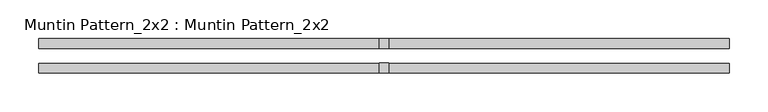
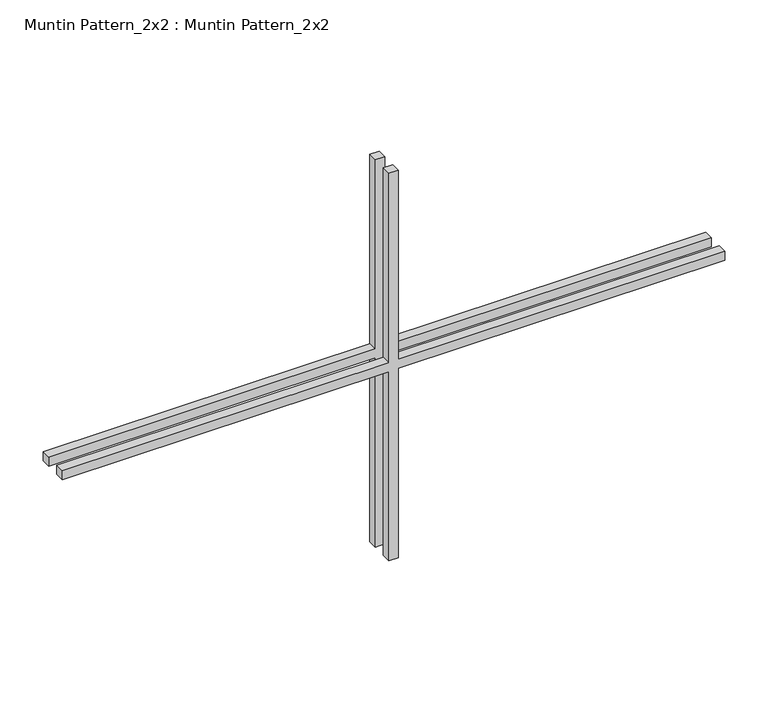
"""IFC4 building model written with IfcOpenShell, lengths in millimetres: proxy geometry, Muntin Pattern_2x2 : Muntin Pattern_2x2."""

from ifc_helpers import new_model, si_unit, frame, origin, place, context, project, spatial, polyline, outline, extrude, source, transform, mapped, element, save


def muntin_pattern_2x2_muntin_pattern_2x2_da9c8da6(model_context):
    return source(origin(), model_context, "Body", "SweptSolid", [
        extrude(outline(polyline([(280.9875, -6.35), (280.9875, -444.5), (268.2875, -444.5), (268.2875, -6.35), (0.0, -6.35), (0.0, 6.35), (268.2875, 6.35), (268.2875, 444.5), (280.9875, 444.5), (280.9875, 6.35), (549.275, 6.35), (549.275, -6.35), (280.9875, -6.35)])), frame((0.0, -22.225, 0.0), z_axis=(0.0, 1.0, 0.0), x_axis=(0.0, 0.0, 1.0)), (0.0, 0.0, 1.0), 12.7),
        extrude(outline(polyline([(280.9875, -6.35), (280.9875, -444.5), (268.2875, -444.5), (268.2875, -6.35), (0.0, -6.35), (0.0, 6.35), (268.2875, 6.35), (268.2875, 444.5), (280.9875, 444.5), (280.9875, 6.35), (549.275, 6.35), (549.275, -6.35), (280.9875, -6.35)])), frame((0.0, 9.525, 0.0), z_axis=(0.0, 1.0, 0.0), x_axis=(0.0, 0.0, 1.0)), (0.0, 0.0, 1.0), 12.7),
    ])


if __name__ == "__main__":
    model = new_model("IFC4")
    model_context = context("Model", 3, world=origin())
    ifc_project = project(units=[si_unit("LENGTHUNIT", "METRE", prefix="MILLI")], contexts=[model_context])
    site = spatial("IfcSite", under=ifc_project)
    building = spatial("IfcBuilding", under=site)
    placement = place(None, origin())
    muntin_pattern_2x2_muntin_pattern_2x2_shape = muntin_pattern_2x2_muntin_pattern_2x2_da9c8da6(model_context)
    element("IfcBuildingElementProxy", 1, Name="Muntin Pattern_2x2 : Muntin Pattern_2x2", ObjectType="Muntin Pattern_2x2 : Muntin Pattern_2x2", at=placement, inside=building, context=model_context, shape_type="MappedRepresentation", body=[
        mapped(muntin_pattern_2x2_muntin_pattern_2x2_shape, transform((0.0, 0.0, 0.0), x_axis=(1.0, 0.0, 0.0), y_axis=(0.0, 1.0, 0.0), z_axis=(0.0, 0.0, 1.0))),
    ])
    save(model, "model.ifc")

# Revit data of these elements
# Type "Muntin Pattern_2x2 : Muntin Pattern_2x2"
#   Width [instance default] = 4' - 0"
#   Thickness = 0' - 0 1/2"
#   Height [instance default] = 4' - 0"
#   Distance = 0' - 0 3/4"
#   Interior Material [instance default] = none
#   Exterior Material [instance default] = none
# Element 1 (IfcBuildingElementProxy, "Muntin Pattern_2x2 : Muntin Pattern_2x2")
#   Width = 2' - 11"
#   Height = 1' - 9 5/8"
#   Interior Material = Wood - Stained
#   Exterior Material = Clad - White
#   Materials on its faces: "Clad - White", "Wood - Stained"
# Materials
#   "Clad - White": class "Wood", colour RGB 242 242 238, transparency 0, Cost = 0
#   "Wood - Stained": class "Wood", colour RGB 224 178 126, transparency 0, Cost = 0
